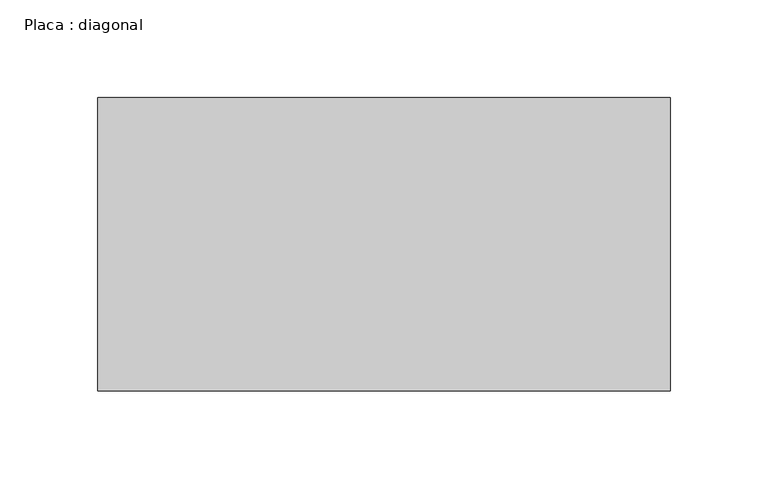
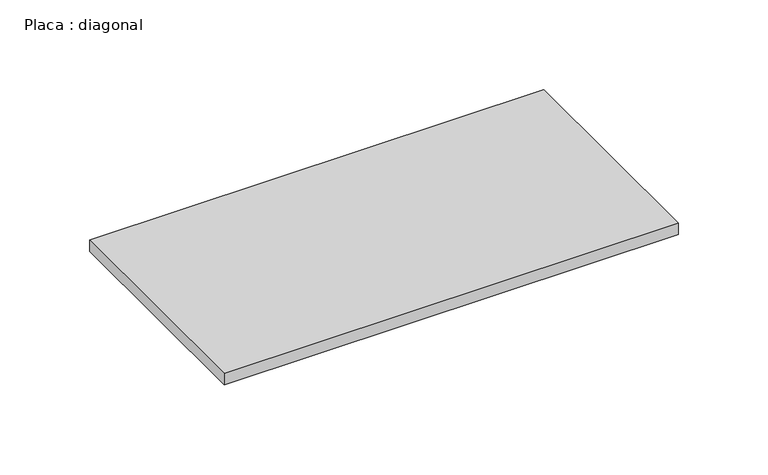
"""IFC4 building model written with IfcOpenShell, lengths in millimetres: beam geometry, Placa : diagonal."""

from ifc_helpers import new_model, si_unit, frame, origin, place, context, project, spatial, polyline, outline, extrude, source, transform, mapped, element, save


def placa_diagonal_a33581f3(model_context):
    return source(origin(), model_context, "Body", "SweptSolid", [
        extrude(outline(polyline([(146.2839954, 75.0), (146.2839954, -75.0), (-146.2743867, -75.0), (-146.2743867, 75.0), (146.2839954, 75.0)])), frame((0.0, 0.0, -4.0), z_axis=(0.0, 0.0, 1.0), x_axis=(1.0, 0.0, 0.0)), (0.0, 0.0, 1.0), 8.0),
    ])


if __name__ == "__main__":
    model = new_model("IFC4")
    model_context = context("Model", 3, world=origin())
    ifc_project = project(units=[si_unit("LENGTHUNIT", "METRE", prefix="MILLI")], contexts=[model_context])
    site = spatial("IfcSite", under=ifc_project)
    building = spatial("IfcBuilding", under=site)
    placement = place(None, origin())
    placa_diagonal_shape = placa_diagonal_a33581f3(model_context)
    element("IfcBeam", 1, ObjectType="Placa : diagonal", at=placement, inside=building, context=model_context, shape_type="MappedRepresentation", body=[
        mapped(placa_diagonal_shape, transform((0.0, 0.0, 0.0), x_axis=(1.0, 0.0, 0.0), y_axis=(0.0, 1.0, 0.0), z_axis=(0.0, 0.0, 1.0))),
    ])
    save(model, "model.ifc")

# Revit data of these elements
# Type "Placa : diagonal"
#   W = 0
#   Length [instance default] = 1.50 m
#   b = 0.15 m
#   d = 0.008 m
#   A = 0 m²
#   Structural Material [instance default] = Aço, 45-345
# Element 1 (IfcBeam, "Placa : diagonal")
#   Materials on its faces: "Aço, 45-345"
# Materials
#   "Aço, 45-345": class "Metal", colour RGB 247 247 247, transparency 0, Description = "Aço 345 MPa", Cost = 0
